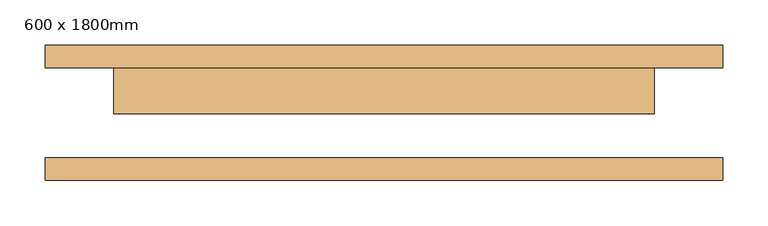
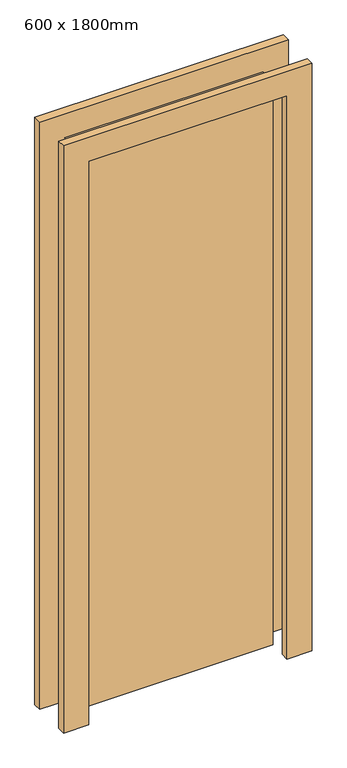
"""IFC4 building model written with IfcOpenShell, lengths in millimetres: door geometry, 单扇 - 与墙齐 : 600 x 1800mm."""

from ifc_helpers import new_model, si_unit, frame, origin, origin_with_axes, place, context, project, spatial, polyline, outline, extrude, source, transform, mapped, element, save


def door_600_x_1800mm_79ebe2d6(model_context):
    return source(origin(), model_context, "Body", "SweptSolid", [
        extrude(outline(polyline([(1876.0, -376.0), (0.0, -376.0), (0.0, -300.0), (1800.0, -300.0), (1800.0, 300.0), (0.0, 300.0), (0.0, 376.0), (1876.0, 376.0), (1876.0, -376.0)])), frame((0.0, 50.0, 0.0), z_axis=(0.0, 1.0, 0.0), x_axis=(0.0, 0.0, 1.0)), (0.0, 0.0, 1.0), 25.0),
        extrude(outline(polyline([(1876.0, 376.0), (1876.0, -376.0), (0.0, -376.0), (0.0, -300.0), (1800.0, -300.0), (1800.0, 300.0), (0.0, 300.0), (0.0, 376.0), (1876.0, 376.0)])), frame((0.0, -75.0, 0.0), z_axis=(0.0, 1.0, 0.0), x_axis=(0.0, 0.0, 1.0)), (0.0, 0.0, 1.0), 25.0),
        extrude(outline(polyline([(300.0, -1.0), (-300.0, -1.0), (-300.0, 50.0), (300.0, 50.0), (300.0, -1.0)])), origin_with_axes(), (0.0, 0.0, 1.0), 1800.0),
    ])


if __name__ == "__main__":
    model = new_model("IFC4")
    model_context = context("Model", 3, world=origin())
    ifc_project = project(units=[si_unit("LENGTHUNIT", "METRE", prefix="MILLI")], contexts=[model_context])
    site = spatial("IfcSite", under=ifc_project)
    building = spatial("IfcBuilding", under=site)
    placement = place(None, origin())
    door_600_x_1800mm_shape = door_600_x_1800mm_79ebe2d6(model_context)
    element("IfcDoor", 1, ObjectType="单扇 - 与墙齐 : 600 x 1800mm", at=placement, inside=building, context=model_context, shape_type="MappedRepresentation", body=[
        mapped(door_600_x_1800mm_shape, transform((0.0, 0.0, 0.0), x_axis=(1.0, 0.0, 0.0), y_axis=(0.0, 1.0, 0.0), z_axis=(0.0, 0.0, 1.0))),
    ])
    save(model, "model.ifc")

# Revit data of these elements
# Type "单扇 - 与墙齐 : 600 x 1800mm"
#   Type Mark = "M0618"
#   Construction Type Id = "MDOOR"
#   Analytic Construction = "金属"
#   贴面宽度 = 76 mm
#   贴面投影内部 = 25 mm
#   贴面投影外部 = 25 mm
#   Thickness = 51 mm
#   Height = 1800 mm
#   Width = 600 mm
#   Heat Transfer Coefficient (U) = 3.7021 W/(m²·K)
#   框架材质 = 门 - 框架
#   门材质 = 门 - 嵌板
#   Visual Light Transmittance = 0
#   Solar Heat Gain Coefficient = 0
#   Wall Closure = (empty or 0)
#   Function = (empty or 0)
# Element 1 (IfcDoor, "单扇 - 与墙齐 : 600 x 1800mm")
#   Materials on its faces: "门 - 框架", "门 - 嵌板"
# Materials
#   "门 - 框架": class "其他", colour RGB 118 70 51, transparency 0, Cost = 0
#   "门 - 嵌板": class "木质", colour RGB 210 159 95, transparency 0, Cost = 0
